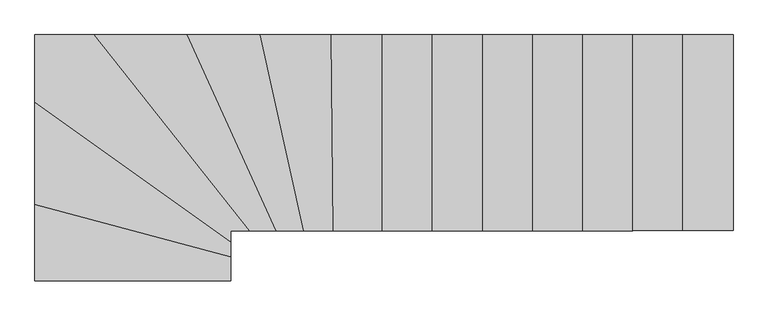
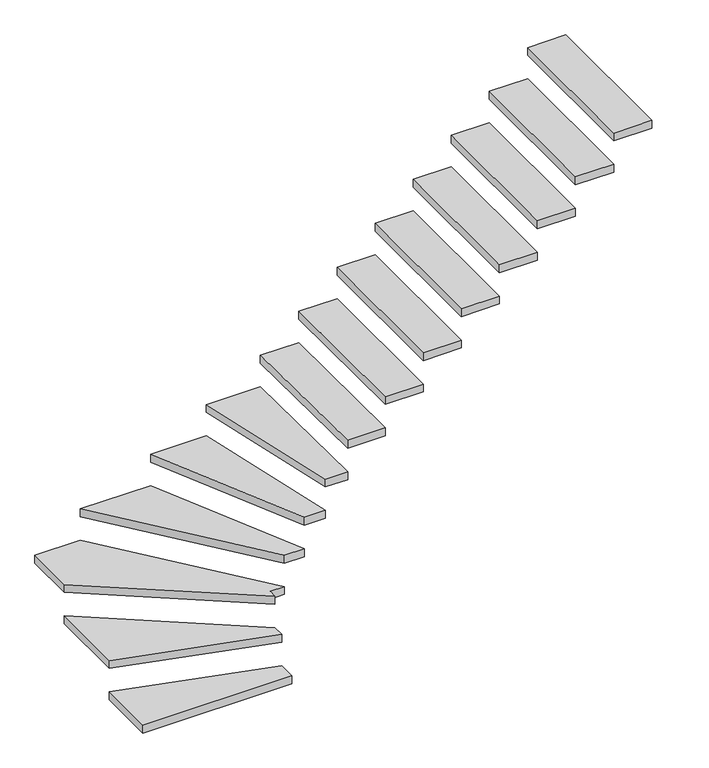
"""IFC4 building model written with IfcOpenShell, lengths in millimetres: stair geometry,   149542 :   149542."""

from ifc_helpers import new_model, si_unit, frame, origin, place, context, project, spatial, polyline, outline, extrude, source, transform, mapped, element, save


def stair_92ba3d55(model_context):
    return source(origin(), model_context, "Body", "SweptSolid", [
        extrude(outline(polyline([(160077.7593015, 32139.1812131), (160077.7593015, 32029.7962965), (159177.7593015, 32029.7962965), (159177.7593015, 32381.5903923), (160077.7593015, 32139.1812131)])), frame((0.0, 0.0, 3480.0), z_axis=(0.0, 0.0, 1.0), x_axis=(1.0, 0.0, 0.0)), (0.0, 0.0, 1.0), 50.0),
        extrude(outline(polyline([(160077.7593015, 32208.6851854), (160077.7593015, 32139.1812131), (159177.7593015, 32381.5903923), (159177.7593015, 32851.1265298), (160077.7593015, 32208.6851854)])), frame((0.0, 0.0, 3680.0), z_axis=(0.0, 0.0, 1.0), x_axis=(1.0, 0.0, 0.0)), (0.0, 0.0, 1.0), 50.0),
        extrude(outline(polyline([(159450.38828, 33159.7962965), (160164.4298971, 32259.7962965), (160077.7593015, 32259.7962965), (160077.7593015, 32208.6851854), (159177.7593015, 32851.1265298), (159177.7593015, 33159.7962965), (159450.38828, 33159.7962965)])), frame((0.0, 0.0, 3880.0), z_axis=(0.0, 0.0, 1.0), x_axis=(1.0, 0.0, 0.0)), (0.0, 0.0, 1.0), 50.0),
        extrude(outline(polyline([(160285.4396784, 32259.7962965), (160164.4298971, 32259.7962965), (159450.38828, 33159.7962965), (159877.5404106, 33159.7962965), (160285.4396784, 32259.7962965)])), frame((0.0, 0.0, 4080.0), z_axis=(0.0, 0.0, 1.0), x_axis=(1.0, 0.0, 0.0)), (0.0, 0.0, 1.0), 50.0),
        extrude(outline(polyline([(160412.2916695, 32259.7962965), (160285.4396784, 32259.7962965), (159877.5404106, 33159.7962965), (160212.4306066, 33159.7962965), (160412.2916695, 32259.7962965)])), frame((0.0, 0.0, 4280.0), z_axis=(0.0, 0.0, 1.0), x_axis=(1.0, 0.0, 0.0)), (0.0, 0.0, 1.0), 50.0),
        extrude(outline(polyline([(160546.5910216, 32259.7962965), (160412.2916695, 32259.7962965), (160212.4306066, 33159.7962965), (160538.1312545, 33159.7962965), (160546.5910216, 32259.7962965)])), frame((0.0, 0.0, 4480.0), z_axis=(0.0, 0.0, 1.0), x_axis=(1.0, 0.0, 0.0)), (0.0, 0.0, 1.0), 50.0),
        extrude(outline(polyline([(160772.3611381, 32259.7962965), (160546.5910216, 32259.7962965), (160538.1312545, 33159.7962965), (160772.3611381, 33159.7962965), (160772.3611381, 32259.7962965)])), frame((0.0, 0.0, 4680.0), z_axis=(0.0, 0.0, 1.0), x_axis=(1.0, 0.0, 0.0)), (0.0, 0.0, 1.0), 50.0),
        extrude(outline(polyline([(161002.3611381, 32259.7962965), (160772.3611381, 32259.7962965), (160772.3611381, 33159.7962965), (161002.3611381, 33159.7962965), (161002.3611381, 32259.7962965)])), frame((0.0, 0.0, 4880.0), z_axis=(0.0, 0.0, 1.0), x_axis=(1.0, 0.0, 0.0)), (0.0, 0.0, 1.0), 50.0),
        extrude(outline(polyline([(161232.3611381, 32259.7962965), (161002.3611381, 32259.7962965), (161002.3611381, 33159.7962965), (161232.3611381, 33159.7962965), (161232.3611381, 32259.7962965)])), frame((0.0, 0.0, 5080.0), z_axis=(0.0, 0.0, 1.0), x_axis=(1.0, 0.0, 0.0)), (0.0, 0.0, 1.0), 50.0),
        extrude(outline(polyline([(161462.3611381, 32259.7962965), (161232.3611381, 32259.7962965), (161232.3611381, 33159.7962965), (161462.3611381, 33159.7962965), (161462.3611381, 32259.7962965)])), frame((0.0, 0.0, 5280.0), z_axis=(0.0, 0.0, 1.0), x_axis=(1.0, 0.0, 0.0)), (0.0, 0.0, 1.0), 50.0),
        extrude(outline(polyline([(161692.3611381, 32259.7962965), (161462.3611381, 32259.7962965), (161462.3611381, 33159.7962965), (161692.3611381, 33159.7962965), (161692.3611381, 32259.7962965)])), frame((0.0, 0.0, 5480.0), z_axis=(0.0, 0.0, 1.0), x_axis=(1.0, 0.0, 0.0)), (0.0, 0.0, 1.0), 50.0),
        extrude(outline(polyline([(161922.3611381, 32259.7962965), (161692.3611381, 32259.7962965), (161692.3611381, 33159.7962965), (161922.3611381, 33159.7962965), (161922.3611381, 32259.7962965)])), frame((0.0, 0.0, 5680.0), z_axis=(0.0, 0.0, 1.0), x_axis=(1.0, 0.0, 0.0)), (0.0, 0.0, 1.0), 50.0),
        extrude(outline(polyline([(162152.3611381, 32259.7962965), (161922.3611381, 32259.7962965), (161922.3611381, 33159.7962965), (162152.3611381, 33159.7962965), (162152.3611381, 32259.7962965)])), frame((0.0, 0.0, 5880.0), z_axis=(0.0, 0.0, 1.0), x_axis=(1.0, 0.0, 0.0)), (0.0, 0.0, 1.0), 50.0),
        extrude(outline(polyline([(162382.3611381, 32259.7962965), (162152.3611381, 32259.7962965), (162152.3611381, 33159.7962965), (162382.3611381, 33159.7962965), (162382.3611381, 32259.7962965)])), frame((0.0, 0.0, 6080.0), z_axis=(0.0, 0.0, 1.0), x_axis=(1.0, 0.0, 0.0)), (0.0, 0.0, 1.0), 50.0),
    ])


if __name__ == "__main__":
    model = new_model("IFC4")
    model_context = context("Model", 3, world=origin())
    ifc_project = project(units=[si_unit("LENGTHUNIT", "METRE", prefix="MILLI")], contexts=[model_context])
    site = spatial("IfcSite", under=ifc_project)
    building = spatial("IfcBuilding", under=site)
    placement = place(None, origin())
    stair_shape = stair_92ba3d55(model_context)
    element("IfcStair", 1, ObjectType="  149542 :   149542", at=placement, inside=building, context=model_context, shape_type="MappedRepresentation", body=[
        mapped(stair_shape, transform((0.0, 0.0, 0.0), x_axis=(1.0, 0.0, 0.0), y_axis=(0.0, 1.0, 0.0), z_axis=(0.0, 0.0, 1.0))),
    ])
    save(model, "model.ifc")

# Revit data of these elements
# Type "  149542 :   149542"
#   Abrechnungsart = "St"
#   Allright_Bauteil_ID = "0131Tre0659044515"
#   Material = "Stahlbeton"
#   Objektname = "Treppe"
#   NameOverride = " "
#   ThermalTransmittance = 0.0000 BTU/(h·ft²·°F)
#   NosingLength = 0.000 m
#   NumberOfRiser = 14
#   NumberOfTreads = 14
#   RiserHeight = 2.000 m
#   TreadLength = 2.300 m
#   IsExternal = no
#   FireExit = no
#   HandicapAccessible = no
#   HasNonSkidSurface = no
# Element 1 (IfcStair, "  149542 :   149542")
#   Materials on its faces: "weiss"
# Materials
#   "weiss": class "Unassigned", colour RGB 255 255 255, transparency 0
